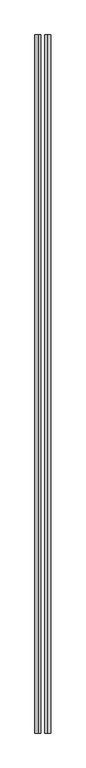
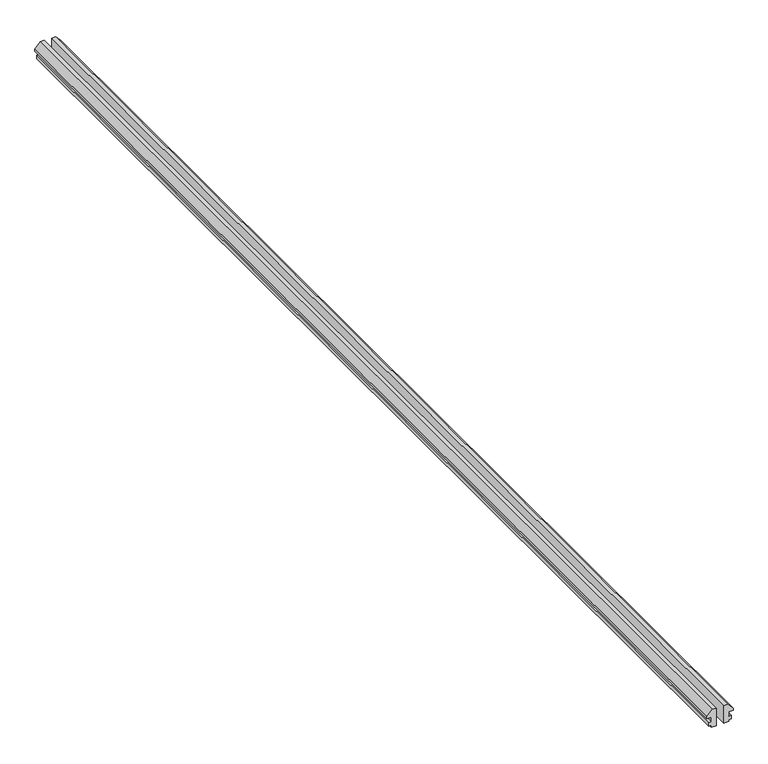
"""IFC4 building model written with IfcOpenShell, lengths in millimetres: proxy geometry, Metal profile084 2060 : Metal profile084 2060."""

import ifcopenshell
import ifcopenshell.guid

model = None  # the IFC model being written
_history = None  # IfcOwnerHistory: only IFC2X3 demands one
_inside = {}  # id of a spatial element -> (the spatial element, [elements in it])
_under = {}  # id of a project, library or spatial element -> (it, [spatial elements below it])
_declared = {}  # id of a project -> (the project, [libraries it declares])
_typed = {}  # id of a type object -> (the type object, [elements of that type])
_made_of = {}  # id of a material, layer set ... -> (it, [elements and type objects made of it])


def new_model(schema):
    """Start an empty IFC model of exactly this schema.

    Asked for "IFC4X3", IfcOpenShell would pick the latest addendum, in which some entities
    have other attributes; the version numbers below select the first issue.
    IFC2X3 requires an IfcOwnerHistory on every rooted entity: one is made here for all.
    """
    global model, _history
    if schema == "IFC4X3":
        model = ifcopenshell.file(schema_version=(4, 3, 0, 0))
    else:
        model = ifcopenshell.file(schema=schema)
    _inside.clear()
    _under.clear()
    _declared.clear()
    _typed.clear()
    _made_of.clear()
    _history = None
    if model.schema == "IFC2X3":
        org = make("IfcOrganization", Name="unknown")
        user = make(
            "IfcPersonAndOrganization",
            ThePerson=make("IfcPerson", FamilyName="unknown"),
            TheOrganization=org,
        )
        app = make(
            "IfcApplication",
            ApplicationDeveloper=org,
            Version="unknown",
            ApplicationFullName="unknown",
            ApplicationIdentifier="unknown",
        )
        _history = make(
            "IfcOwnerHistory",
            OwningUser=user,
            OwningApplication=app,
            ChangeAction="ADDED",
            CreationDate=0,
        )
    return model


def make(cls, **values):
    """One entity of the class cls with the attributes given. An attribute that is None is left unset."""
    return model.create_entity(
        cls, **{name: value for name, value in values.items() if value is not None}
    )


def rooted(cls, **values):
    """An entity with a GlobalId (a new one), such as an element, a storey or a relation."""
    return make(cls, GlobalId=ifcopenshell.guid.new(), OwnerHistory=_history, **values)


def si_unit(unit_type, name, prefix=None):
    """IfcSIUnit, for example si_unit("LENGTHUNIT", "METRE", prefix="MILLI")."""
    return make("IfcSIUnit", UnitType=unit_type, Prefix=prefix, Name=name)


def assignment(units):
    """IfcUnitAssignment: the units of a project."""
    return None if units is None else make("IfcUnitAssignment", Units=units)


def point(xyz):
    """IfcCartesianPoint."""
    return None if xyz is None else make("IfcCartesianPoint", Coordinates=xyz)


def direction(xyz):
    """IfcDirection."""
    return None if xyz is None else make("IfcDirection", DirectionRatios=xyz)


def frame(location, z_axis=None, x_axis=None):
    """IfcAxis2Placement3D, a coordinate frame: its origin and axes. An axis left out is left unset."""
    return make(
        "IfcAxis2Placement3D",
        Location=point(location),
        Axis=direction(z_axis),
        RefDirection=direction(x_axis),
    )


def origin():
    """The frame at (0, 0, 0) with its axes left unset."""
    return frame((0.0, 0.0, 0.0))


def place(relative_to, where):
    """IfcLocalPlacement: puts the frame where relative to a parent placement (None: the world)."""
    return make(
        "IfcLocalPlacement", PlacementRelTo=relative_to, RelativePlacement=where
    )


def context(
    kind, dimensions, precision=None, world=None, true_north=None, identifier=None
):
    """IfcGeometricRepresentationContext, for example the 3D "Model" context."""
    return make(
        "IfcGeometricRepresentationContext",
        ContextIdentifier=identifier,
        ContextType=kind,
        CoordinateSpaceDimension=dimensions,
        Precision=precision,
        WorldCoordinateSystem=world,
        TrueNorth=true_north,
    )


def project(units=None, contexts=None):
    """IfcProject with its units and contexts."""
    return rooted(
        "IfcProject",
        Name="project",
        RepresentationContexts=contexts,
        UnitsInContext=assignment(units),
    )


def spatial(cls, under=None, at=None, **own):
    """A site, building, storey or space (cls), placed at a placement, below another one or the project."""
    s = rooted(cls, ObjectPlacement=at, **own)
    if under is not None:
        _under.setdefault(under.id(), (under, []))[1].append(s)
    return s


def polyline(points):
    """IfcPolyline through the points."""
    return make("IfcPolyline", Points=[point(p) for p in points])


def outline(outer, holes=None, kind="AREA"):
    """IfcArbitraryClosedProfileDef: a profile drawn as a closed curve; with holes, ...WithVoids."""
    if holes is None:
        return make("IfcArbitraryClosedProfileDef", ProfileType=kind, OuterCurve=outer)
    return make(
        "IfcArbitraryProfileDefWithVoids",
        ProfileType=kind,
        OuterCurve=outer,
        InnerCurves=holes,
    )


def extrude(swept, where, along, depth):
    """IfcExtrudedAreaSolid: the profile swept, set in the frame where, extruded along a direction by depth."""
    return make(
        "IfcExtrudedAreaSolid",
        SweptArea=swept,
        Position=where,
        ExtrudedDirection=direction(along),
        Depth=depth,
    )


def shape(context_of_items, identifier, shape_type, items):
    """IfcShapeRepresentation: the items that make up one representation, for example the "Body"."""
    return make(
        "IfcShapeRepresentation",
        ContextOfItems=context_of_items,
        RepresentationIdentifier=identifier,
        RepresentationType=shape_type,
        Items=items,
    )


def source(mapping_origin, context_of_items, identifier, shape_type, items):
    """IfcRepresentationMap: a shape defined once, which mapped items show again and again."""
    return make(
        "IfcRepresentationMap",
        MappingOrigin=mapping_origin,
        MappedRepresentation=shape(context_of_items, identifier, shape_type, items),
    )


def transform(
    local_origin,
    x_axis=None,
    y_axis=None,
    z_axis=None,
    scale=None,
    scale2=None,
    scale3=None,
    uniform=True,
):
    """IfcCartesianTransformationOperator3D, or its non-uniform kind. x_axis, y_axis, z_axis: its Axis1, 2, 3."""
    if uniform:
        return make(
            "IfcCartesianTransformationOperator3D",
            Axis1=direction(x_axis),
            Axis2=direction(y_axis),
            LocalOrigin=point(local_origin),
            Scale=scale,
            Axis3=direction(z_axis),
        )
    return make(
        "IfcCartesianTransformationOperator3DnonUniform",
        Axis1=direction(x_axis),
        Axis2=direction(y_axis),
        LocalOrigin=point(local_origin),
        Scale=scale,
        Axis3=direction(z_axis),
        Scale2=scale2,
        Scale3=scale3,
    )


def mapped(mapping_source, mapping_target):
    """IfcMappedItem: shows the shape of a source again, moved by a transform."""
    return make(
        "IfcMappedItem", MappingSource=mapping_source, MappingTarget=mapping_target
    )


def made_of(thing, what):
    """Note that an element or type object is made of a material, layer set ...; save() writes the relation."""
    if what is not None:
        _made_of.setdefault(what.id(), (what, []))[1].append(thing)
    return thing


def element(
    cls,
    number,
    at=None,
    inside=None,
    cuts=None,
    type_object=None,
    material=None,
    context=None,
    identifier="Body",
    shape_type=None,
    held_by="IfcProductDefinitionShape",
    body=None,
    shapes=None,
    **own,
):
    """One element of the class cls, such as IfcWall. Its Tag is "e" and its number.

    at: its placement. inside: the storey or other place that contains it. cuts: it is an
    opening in that element (IfcRelVoidsElement). A single representation is given by context,
    identifier, shape_type and body (its items); several are given by shapes. held_by: the class
    of the entity that holds the representations. save() writes the other relations.
    """
    e = rooted(cls, Tag="e%d" % number, ObjectPlacement=at, **own)
    if body is not None:
        shapes = [shape(context, identifier, shape_type, body)]
    if shapes is not None:
        e.Representation = make(held_by, Representations=shapes)
    if inside is not None:
        _inside.setdefault(inside.id(), (inside, []))[1].append(e)
    if cuts is not None:
        rooted(
            "IfcRelVoidsElement", RelatingBuildingElement=cuts, RelatedOpeningElement=e
        )
    if type_object is not None:
        _typed.setdefault(type_object.id(), (type_object, []))[1].append(e)
    return made_of(e, material)


def aggregate(whole, parts):
    """IfcRelAggregates: a whole, such as a stair, and the parts it consists of."""
    return rooted("IfcRelAggregates", RelatingObject=whole, RelatedObjects=parts)


def save(model, path):
    """Write the relations noted so far, then the file.

    IfcRelAggregates (storeys below a building ...), IfcRelContainedInSpatialStructure (elements
    in a storey), IfcRelDefinesByType, IfcRelAssociatesMaterial and IfcRelDeclares: one each for
    every whole, place, type object, material and project.
    """
    for whole, parts in _under.values():
        aggregate(whole, parts)
    for where, things in _inside.values():
        rooted(
            "IfcRelContainedInSpatialStructure",
            RelatedElements=things,
            RelatingStructure=where,
        )
    for kind, things in _typed.values():
        rooted("IfcRelDefinesByType", RelatedObjects=things, RelatingType=kind)
    for what, things in _made_of.values():
        rooted("IfcRelAssociatesMaterial", RelatedObjects=things, RelatingMaterial=what)
    for by, libraries in _declared.values():
        rooted("IfcRelDeclares", RelatingContext=by, RelatedDefinitions=libraries)
    model.write(path)


def generic_models_66654635(model_context):
    return source(origin(), model_context, "Body", "SweptSolid", [
        extrude(outline(polyline([(40189.149371, -7057.8334674), (40192.2147583, -7057.8334674), (40192.2147583, -7053.304964), (40198.9413208, -7053.304964), (40198.9413208, -7057.8334674), (40207.2092895, -7057.8334674), (40207.2092895, -7050.0896497), (40210.5517148, -7050.0896497), (40220.8759335, -7059.3926282), (40220.8759335, -7066.2334918), (40189.149371, -7066.2334918), (40189.149371, -7057.8334674)])), frame((0.0, 7182.1531721, 0.0), z_axis=(0.0, 1.0, 0.0), x_axis=(0.0, 0.0, 1.0)), (0.0, 0.0, 1.0), 2000.0),
        extrude(outline(polyline([(40189.149371, -7087.3335162), (40189.149371, -7078.9334918), (40220.8759335, -7078.9334918), (40220.8759335, -7085.7743555), (40210.5517148, -7095.077334), (40207.2092895, -7095.077334), (40207.2092895, -7087.3335162), (40198.9413208, -7087.3335162), (40198.9413208, -7091.8620197), (40192.2147583, -7091.8620197), (40192.2147583, -7087.3335162), (40189.149371, -7087.3335162)])), frame((0.0, 7182.1531721, 0.0), z_axis=(0.0, 1.0, 0.0), x_axis=(0.0, 0.0, 1.0)), (0.0, 0.0, 1.0), 2000.0),
    ])


if __name__ == "__main__":
    model = new_model("IFC4")
    model_context = context("Model", 3, world=origin())
    ifc_project = project(units=[si_unit("LENGTHUNIT", "METRE", prefix="MILLI")], contexts=[model_context])
    site = spatial("IfcSite", under=ifc_project)
    building = spatial("IfcBuilding", under=site)
    placement = place(None, origin())
    generic_models_shape = generic_models_66654635(model_context)
    element("IfcBuildingElementProxy", 1, Name="Metal profile084 2060 : Metal profile084 2060", ObjectType="Metal profile084 2060 : Metal profile084 2060", at=placement, inside=building, context=model_context, shape_type="MappedRepresentation", body=[
        mapped(generic_models_shape, transform((0.0, 0.0, 0.0), x_axis=(1.0, 0.0, 0.0), y_axis=(0.0, 1.0, 0.0), z_axis=(0.0, 0.0, 1.0))),
    ])
    save(model, "model.ifc")

# Revit data of these elements
# Type "Metal profile084 2060 : Metal profile084 2060"
#   NameOverride = "Metal profile084"
# Element 1 (IfcBuildingElementProxy, "Metal profile084 2060 : Metal profile084 2060")
#   Materials on its faces: "RUBBER GASKET"
# Materials
#   "RUBBER GASKET": class "Unassigned", colour RGB 70 70 70, transparency 0
